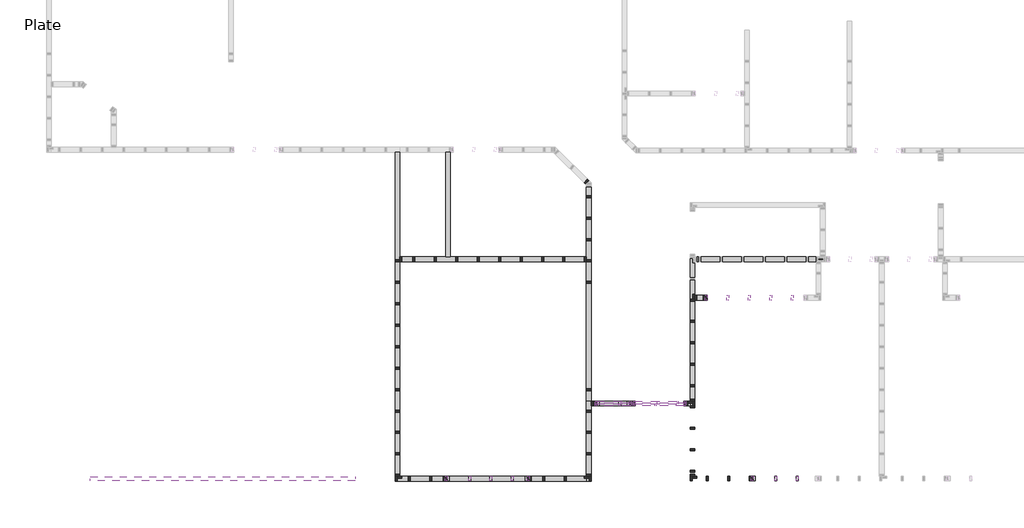
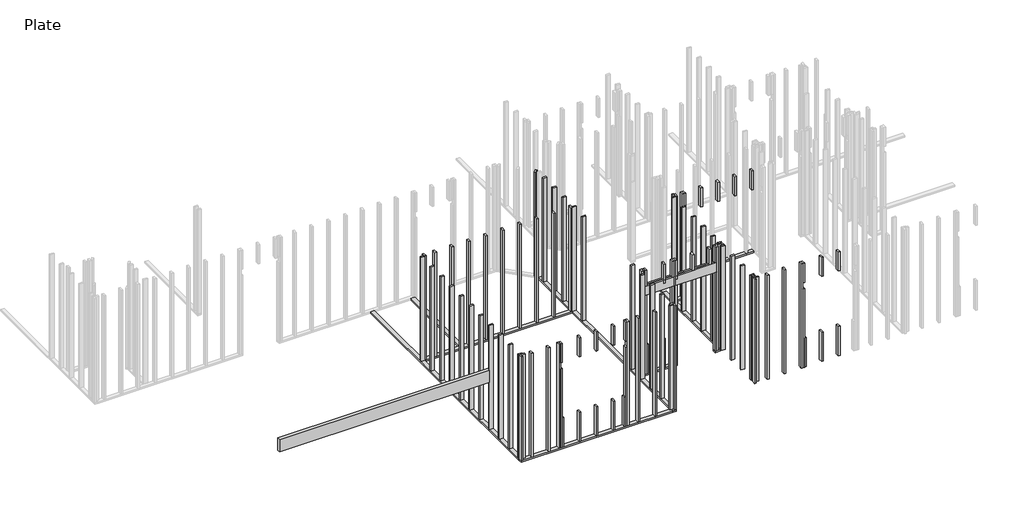
# One storey, part 1 of 5: 106 columns, 16 beams.
# Revit data of these elements (continued)
# Type "Dimension Lumber : 2x10 Header Exterior"
#   Assembly Code = "B10"
#   A = 0.0963889 SF
#   Length [instance default] = 5' - 0"
#   b = 0' - 1 1/2"
#   d = 0' - 9 1/4"
#   Structural Material [instance default] = Softwood, Lumber
# Type "Dimension Lumber : 2x10 Header Interior"
#   Assembly Code = "B10"
#   A = 0.0963889 SF
#   Length [instance default] = 5' - 0"
#   b = 0' - 1 1/2"
#   d = 0' - 9 1/4"
#   Structural Material [instance default] = Softwood, Lumber
# Type "Dimension Lumber : Supporting Bottom Plate"
#   Assembly Code = "B10"
#   A = 0.0364583 SF
#   Length [instance default] = 5' - 0"
#   b = 0' - 3 1/2"
#   d = 0' - 1 1/2"
#   Structural Material [instance default] = Softwood, Lumber
# Type "Glulam-Western Species : 3.125x12 Headers Exterior"
#   Assembly Code = "B10"
#   Laminations = "8"
#   A = 0.260417 SF
#   Ix = 450
#   Iy = 30.52
#   Length [instance default] = 5' - 0"
#   Sx = 75
#   Sy = 19.53
#   b = 0' - 3 1/8"
#   d = 1' - 0"
#   Structural Material [instance default] = Softwood, Lumber
# Type "Dimension Lumber-Column : 2x4"
#   Int Type = "Interior"
#   Assembly Code = "B10"
#   Cost = 8.05
#   A = 0.0364583 SF
#   b = 0' - 1 1/2"
#   d = 0' - 3 1/2"
#   Structural Material [instance default] = Softwood, Lumber
# Elements 1, 2 (IfcBeam, "Dimension Lumber : 2x10 Header Exterior")
#   Comments = ""
#   Structural Material = Douglas Fir #2
#   Phase Created = New Construction
#   Materials on its faces: "Douglas Fir #2"
# Elements 3, 4 (IfcBeam, "Dimension Lumber : 2x10 Header Interior")
#   Comments = ""
#   Structural Material = Douglas Fir #2
#   Phase Created = New Construction
#   Materials on its faces: "Douglas Fir #2"
# Elements 5, 6, 7, 8, 9, 10, 12, 13, 14, 15 (IfcBeam, "Dimension Lumber : Supporting Bottom Plate")
#   Structural Material = Douglas Fir #2
#   Phase Created = New Construction
#   Materials on its faces: "Douglas Fir #2"
# Element 11 (IfcBeam, "Dimension Lumber : Supporting Bottom Plate")
#   Comments = ""
#   Structural Material = Douglas Fir #2
#   Phase Created = New Construction
#   Materials on its faces: "Douglas Fir #2"
# Element 16 (IfcBeam, "Glulam-Western Species : 3.125x12 Headers Exterior")
#   Comments = ""
#   Structural Material = Douglas Fir #2
#   Phase Created = New Construction
#   Materials on its faces: "Douglas Fir #2"
# Elements 17, 18, 19, 20, 21, 22, 23, 24, 25, 26, 27, 28, 29, 30, 31, 33, 34, 36, 37, 49, 53, 54, 55, 56, 57, 64, 81, 82, 83, 84, 85, 86, 87, 89, 90, 91, 92, 93, 94, 95, 96, 97, 98, 99, 100, 101, 102, 103 (IfcColumn, "Dimension Lumber-Column : 2x4")
#   Function = "Exterior"
#   Structural Material = Douglas Fir #2
#   Phase Created = New Construction
#   Materials on its faces: "Douglas Fir #2"
# Elements 32, 35, 38, 39, 40, 41, 42, 43, 44, 45, 46, 47, 48, 50, 51, 52, 58, 59, 60, 61, 62, 63, 65, 66, 67, 68, 69, 70, 71, 72, 73, 74, 75, 76, 77, 78, 79, 80, 88, 104, 105, 106, 107, 108 (IfcColumn, "Dimension Lumber-Column : 2x4")
#   Function = "Interior"
#   Structural Material = Douglas Fir #2
#   Phase Created = New Construction
#   Materials on its faces: "Douglas Fir #2"
# Elements 109, 110, 111, 112, 113, 114, 115, 116, 117, 118, 119 (IfcColumn, "Dimension Lumber-Column : 2x4")
#   Structural Material = Douglas Fir #2
#   Phase Created = New Construction
#   Materials on its faces: "Douglas Fir #2"
# Elements 120, 121, 122 (IfcColumn, "Dimension Lumber-Column : 2x4")
#   Function = "Exterior"
#   Structural Material = Softwood, Lumber
#   Phase Created = New Construction
#   Materials on its faces: "Softwood, Lumber"
# Materials
#   "Softwood, Lumber": class "Wood", colour RGB 223 192 134, transparency 0, Description = "Pinus Echinata", Cost = 0
#   "Douglas Fir #2": class "Wood", colour RGB 223 192 134, transparency 0, Description = "Pinus Echinata", Cost = 0
